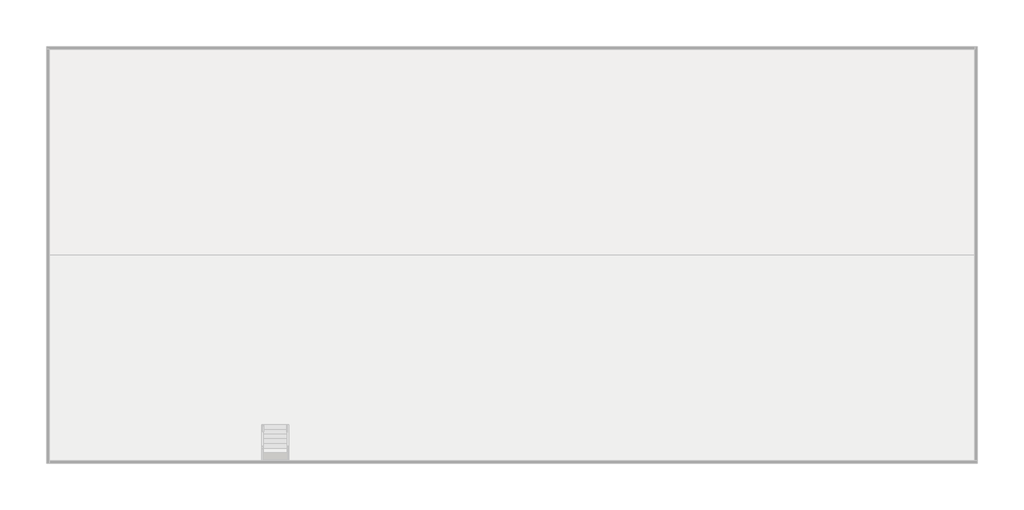
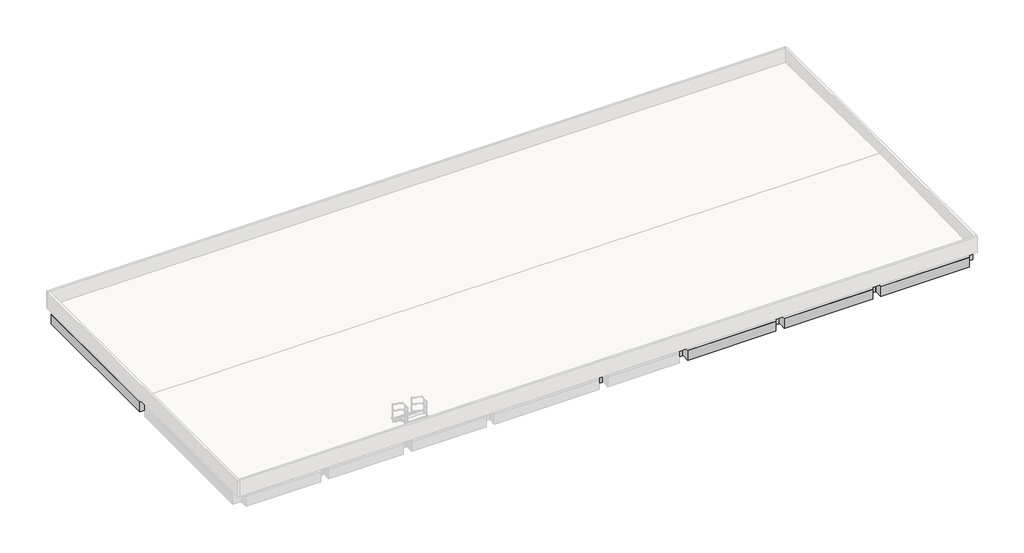
# One storey, part 2 of 3: 33 beams.
"""IFC4 building model written with IfcOpenShell, lengths in millimetres."""

from ifc_helpers import new_model, si_unit, origin, place, context, project, spatial, faceted_brep, element, save

model = new_model("IFC4")

# Units and contexts
model_context = context("Model", 3, world=origin())
ifc_project = project(units=[si_unit("LENGTHUNIT", "METRE", prefix="MILLI")], contexts=[model_context])

# Site, building, storey
site = spatial("IfcSite", under=ifc_project)
building = spatial("IfcBuilding", under=site)
storey = spatial("IfcBuildingStorey", under=building, Name="TOC", Elevation=7499.9618634)

# Beams
placement = place(None, origin())
element("IfcBeam", 1, ObjectType="RC Beam_Rectangular : H_SB_AR_S16_B600xH900_RG9", at=placement, inside=storey, context=model_context, shape_type="Brep", body=[
    faceted_brep([(300.0, 24199.5208589, 6599.9618634), (300.0, 23749.5208589, 6599.9618634), (300.0, 23599.5208589, 6599.9618634), (300.0, 23599.5208589, 7349.9618634), (300.0, 24199.5208589, 7349.9618634), (5700.0, 23599.5208589, 6599.9618634), (5700.0, 23749.5208589, 6599.9618634), (5700.0, 24199.5208589, 6599.9618634), (5700.0, 24199.5208589, 7349.9618634), (5700.0, 23599.5208589, 7349.9618634), (2800.0, 23599.5208589, 7349.9618634), (3200.0, 23599.5208589, 7349.9618634), (2800.0, 23599.5208589, 6599.9618634), (3200.0, 23599.5208589, 6599.9618634)], [[[0, 1, 2, 3, 4]], [[5, 6, 7, 8, 9]], [[4, 3, 10, 11, 9, 8]], [[2, 12, 13, 5, 9, 11, 10, 3]], [[2, 1, 0, 7, 6, 5, 13, 12]], [[7, 0, 4, 8]]]),
])
element("IfcBeam", 2, ObjectType="RC Beam_Rectangular : H_SB_AR_S16_B600xH900_RG9", at=placement, inside=storey, context=model_context, shape_type="Brep", body=[
    faceted_brep([(6300.0, 24199.5208589, 6599.9618634), (6300.0, 23749.5208589, 6599.9618634), (6300.0, 23599.5208589, 6599.9618634), (6300.0, 23599.5208589, 7349.9618634), (6300.0, 24199.5208589, 7349.9618634), (11700.0, 23599.5208589, 6599.9618634), (11700.0, 23749.5208589, 6599.9618634), (11700.0, 24199.5208589, 6599.9618634), (11700.0, 24199.5208589, 7349.9618634), (11700.0, 23599.5208589, 7349.9618634), (8800.0, 23599.5208589, 7349.9618634), (9200.0, 23599.5208589, 7349.9618634), (8800.0, 23599.5208589, 6599.9618634), (9200.0, 23599.5208589, 6599.9618634)], [[[0, 1, 2, 3, 4]], [[5, 6, 7, 8, 9]], [[4, 3, 10, 11, 9, 8]], [[2, 12, 13, 5, 9, 11, 10, 3]], [[2, 1, 0, 7, 6, 5, 13, 12]], [[7, 0, 4, 8]]]),
])
element("IfcBeam", 3, ObjectType="RC Beam_Rectangular : H_SB_AR_S16_B600xH900_RG9", at=placement, inside=storey, context=model_context, shape_type="Brep", body=[
    faceted_brep([(12300.0, 24199.5208589, 6599.9618634), (12300.0, 23749.5208589, 6599.9618634), (12300.0, 23599.5208589, 6599.9618634), (12300.0, 23599.5208589, 7349.9618634), (12300.0, 24199.5208589, 7349.9618634), (17700.0, 23599.5208589, 6599.9618634), (17700.0, 23749.5208589, 6599.9618634), (17700.0, 24199.5208589, 6599.9618634), (17700.0, 24199.5208589, 7349.9618634), (17700.0, 23599.5208589, 7349.9618634), (14800.0, 23599.5208589, 7349.9618634), (15200.0, 23599.5208589, 7349.9618634), (14800.0, 23599.5208589, 6599.9618634), (15200.0, 23599.5208589, 6599.9618634)], [[[0, 1, 2, 3, 4]], [[5, 6, 7, 8, 9]], [[4, 3, 10, 11, 9, 8]], [[2, 12, 13, 5, 9, 11, 10, 3]], [[2, 1, 0, 7, 6, 5, 13, 12]], [[7, 0, 4, 8]]]),
])
element("IfcBeam", 4, ObjectType="RC Beam_Rectangular : H_SB_AR_S16_B600xH900_RG9", at=placement, inside=storey, context=model_context, shape_type="Brep", body=[
    faceted_brep([(18300.0, 24199.5208589, 6599.9618634), (18300.0, 23749.5208589, 6599.9618634), (18300.0, 23599.5208589, 6599.9618634), (18300.0, 23599.5208589, 7349.9618634), (18300.0, 24199.5208589, 7349.9618634), (25900.0, 23599.5208589, 6599.9618634), (25900.0, 23749.5208589, 6599.9618634), (25900.0, 24199.5208589, 6599.9618634), (25900.0, 24199.5208589, 7349.9618634), (25900.0, 23599.5208589, 7349.9618634), (21800.0, 23599.5208589, 7349.9618634), (22400.0, 23599.5208589, 7349.9618634), (21800.0, 23599.5208589, 6599.9618634), (22400.0, 23599.5208589, 6599.9618634)], [[[0, 1, 2, 3, 4]], [[5, 6, 7, 8, 9]], [[4, 3, 10, 11, 9, 8]], [[2, 12, 13, 5, 9, 11, 10, 3]], [[2, 1, 0, 7, 6, 5, 13, 12]], [[7, 0, 4, 8]]]),
])
element("IfcBeam", 5, ObjectType="RC Beam_Rectangular : H_SB_AR_S16_B600xH900_RG9", at=placement, inside=storey, context=model_context, shape_type="Brep", body=[
    faceted_brep([(26500.0, 24199.5208589, 6599.9618634), (26500.0, 23749.5208589, 6599.9618634), (26500.0, 23599.5208589, 6599.9618634), (26500.0, 23599.5208589, 7349.9618634), (26500.0, 24199.5208589, 7349.9618634), (31700.0, 23599.5208589, 6599.9618634), (31700.0, 23749.5208589, 6599.9618634), (31700.0, 24199.5208589, 6599.9618634), (31700.0, 24199.5208589, 7349.9618634), (31700.0, 23599.5208589, 7349.9618634), (28800.0, 23599.5208589, 7349.9618634), (29400.0, 23599.5208589, 7349.9618634), (28800.0, 23599.5208589, 6599.9618634), (29400.0, 23599.5208589, 6599.9618634)], [[[0, 1, 2, 3, 4]], [[5, 6, 7, 8, 9]], [[4, 3, 10, 11, 9, 8]], [[2, 12, 13, 5, 9, 11, 10, 3]], [[2, 1, 0, 7, 6, 5, 13, 12]], [[7, 0, 4, 8]]]),
])
element("IfcBeam", 6, ObjectType="RC Beam_Rectangular : H_SB_AR_S16_B600xH900_RG5", at=placement, inside=storey, context=model_context, shape_type="Brep", body=[
    faceted_brep([(26500.0, 8599.5208589, 6599.9618634), (26500.0, 8399.5208589, 6599.9618634), (26500.0, 7999.5208589, 6599.9618634), (26500.0, 7999.5208589, 7349.9618634), (26500.0, 8599.5208589, 7349.9618634), (31700.0, 7999.5208589, 6599.9618634), (31700.0, 8399.5208589, 6599.9618634), (31700.0, 8599.5208589, 6599.9618634), (31700.0, 8599.5208589, 7349.9618634), (31700.0, 7999.5208589, 7349.9618634), (28500.0, 7999.5208589, 7349.9618634), (28700.0, 7999.5208589, 7349.9618634), (28800.0, 7999.5208589, 7349.9618634), (29400.0, 7999.5208589, 7349.9618634), (29400.0, 8599.5208589, 7349.9618634), (28800.0, 8599.5208589, 7349.9618634), (28500.0, 7999.5208589, 6599.9618634), (28700.0, 7999.5208589, 6599.9618634), (28800.0, 7999.5208589, 6599.9618634), (29400.0, 7999.5208589, 6599.9618634), (28800.0, 8599.5208589, 6599.9618634), (29400.0, 8599.5208589, 6599.9618634)], [[[0, 1, 2, 3, 4]], [[5, 6, 7, 8, 9]], [[4, 3, 10, 11, 12, 13, 9, 8, 14, 15]], [[2, 16, 17, 18, 19, 5, 9, 13, 12, 11, 10, 3]], [[2, 1, 0, 20, 21, 7, 6, 5, 19, 18, 17, 16]], [[7, 21, 20, 0, 4, 15, 14, 8]]]),
])
element("IfcBeam", 7, ObjectType="RC Beam_Rectangular : H_SB_AR_S16_B600xH900_RG5", at=placement, inside=storey, context=model_context, shape_type="Brep", body=[
    faceted_brep([(32300.0, 8599.5208589, 6599.9618634), (32300.0, 8399.5208589, 6599.9618634), (32300.0, 7999.5208589, 6599.9618634), (32300.0, 7999.5208589, 7349.9618634), (32300.0, 8599.5208589, 7349.9618634), (38700.0, 7999.5208589, 6599.9618634), (38700.0, 8599.5208589, 6599.9618634), (38700.0, 8599.5208589, 7349.9618634), (38700.0, 7999.5208589, 7349.9618634), (35200.0, 7999.5208589, 7349.9618634), (35800.0, 7999.5208589, 7349.9618634), (36500.0, 7999.5208589, 7349.9618634), (36700.0, 7999.5208589, 7349.9618634), (36700.0, 8599.5208589, 7349.9618634), (36500.0, 8599.5208589, 7349.9618634), (35800.0, 8599.5208589, 7349.9618634), (35200.0, 8599.5208589, 7349.9618634), (33450.0, 8599.5208589, 7349.9618634), (33250.0, 8599.5208589, 7349.9618634), (35200.0, 7999.5208589, 6599.9618634), (35800.0, 7999.5208589, 6599.9618634), (36500.0, 7999.5208589, 6599.9618634), (36700.0, 7999.5208589, 6599.9618634), (35200.0, 8599.5208589, 6599.9618634), (35800.0, 8599.5208589, 6599.9618634), (36500.0, 8599.5208589, 6599.9618634), (36700.0, 8599.5208589, 6599.9618634)], [[[0, 1, 2, 3, 4]], [[5, 6, 7, 8]], [[4, 3, 9, 10, 11, 12, 8, 7, 13, 14, 15, 16, 17, 18]], [[2, 19, 20, 21, 22, 5, 8, 12, 11, 10, 9, 3]], [[2, 1, 0, 23, 24, 25, 26, 6, 5, 22, 21, 20, 19]], [[6, 26, 25, 24, 23, 0, 4, 18, 17, 16, 15, 14, 13, 7]]]),
])
element("IfcBeam", 8, ObjectType="RC Beam_Rectangular : H_SB_AR_S16_B600xH900_RG5", at=placement, inside=storey, context=model_context, shape_type="Brep", body=[
    faceted_brep([(39300.0, 8599.5208589, 6599.9618634), (39300.0, 8404.5208589, 6599.9618634), (39300.0, 8204.5208589, 6599.9618634), (39300.0, 7999.5208589, 6599.9618634), (39300.0, 7999.5208589, 7349.9618634), (39300.0, 8599.5208589, 7349.9618634), (45700.0, 7999.5208589, 6599.9618634), (45700.0, 8399.5208589, 6599.9618634), (45700.0, 8599.5208589, 6599.9618634), (45700.0, 8599.5208589, 7349.9618634), (45700.0, 7999.5208589, 7349.9618634), (41925.0, 7999.5208589, 7349.9618634), (42125.0, 7999.5208589, 7349.9618634), (42200.0, 7999.5208589, 7349.9618634), (42800.0, 7999.5208589, 7349.9618634), (43200.0, 7999.5208589, 7349.9618634), (43400.0, 7999.5208589, 7349.9618634), (42800.0, 8599.5208589, 7349.9618634), (42200.0, 8599.5208589, 7349.9618634), (41925.0, 7999.5208589, 6599.9618634), (42125.0, 7999.5208589, 6599.9618634), (42200.0, 7999.5208589, 6599.9618634), (42800.0, 7999.5208589, 6599.9618634), (43200.0, 7999.5208589, 6599.9618634), (43400.0, 7999.5208589, 6599.9618634), (42200.0, 8599.5208589, 6599.9618634), (42800.0, 8599.5208589, 6599.9618634), (45640.0, 8599.5208589, 6599.9618634)], [[[0, 1, 2, 3, 4, 5]], [[6, 7, 8, 9, 10]], [[5, 4, 11, 12, 13, 14, 15, 16, 10, 9, 17, 18]], [[3, 19, 20, 21, 22, 23, 24, 6, 10, 16, 15, 14, 13, 12, 11, 4]], [[3, 2, 1, 0, 25, 26, 27, 8, 7, 6, 24, 23, 22, 21, 20, 19]], [[8, 27, 26, 25, 0, 5, 18, 17, 9]]]),
])
element("IfcBeam", 9, ObjectType="RC Beam_Rectangular : H_SB_AR_S16_B600xH900_RG5", at=placement, inside=storey, context=model_context, shape_type="Brep", body=[
    faceted_brep([(46300.0, 8599.5208589, 6599.9618634), (46300.0, 8399.5208589, 6599.9618634), (46300.0, 7999.5208589, 6599.9618634), (46300.0, 7999.5208589, 7349.9618634), (46300.0, 8599.5208589, 7349.9618634), (52700.0, 7999.5208589, 6599.9618634), (52700.0, 8399.5208589, 6599.9618634), (52700.0, 8599.5208589, 6599.9618634), (52700.0, 8599.5208589, 7349.9618634), (52700.0, 7999.5208589, 7349.9618634), (49200.0, 7999.5208589, 7349.9618634), (49800.0, 7999.5208589, 7349.9618634), (52574.0, 7999.5208589, 7349.9618634), (52574.0, 8599.5208589, 7349.9618634), (50725.0, 8599.5208589, 7349.9618634), (50525.0, 8599.5208589, 7349.9618634), (49800.0, 8599.5208589, 7349.9618634), (49200.0, 8599.5208589, 7349.9618634), (49200.0, 7999.5208589, 6599.9618634), (49800.0, 7999.5208589, 6599.9618634), (52574.0, 7999.5208589, 6599.9618634), (49200.0, 8599.5208589, 6599.9618634), (49800.0, 8599.5208589, 6599.9618634)], [[[0, 1, 2, 3, 4]], [[5, 6, 7, 8, 9]], [[4, 3, 10, 11, 12, 9, 8, 13, 14, 15, 16, 17]], [[2, 18, 19, 20, 5, 9, 12, 11, 10, 3]], [[2, 1, 0, 21, 22, 7, 6, 5, 20, 19, 18]], [[7, 22, 21, 0, 4, 17, 16, 15, 14, 13, 8]]]),
])
element("IfcBeam", 10, ObjectType="RC Beam_Rectangular : H_SB_AR_S16_B600xH900_RG9", at=placement, inside=storey, context=model_context, shape_type="Brep", body=[
    faceted_brep([(32300.0, 799.5208589, 6599.9618634), (32300.0, 649.5208589, 6599.9618634), (32300.0, 199.5208589, 6599.9618634), (32300.0, 199.5208589, 7349.9618634), (32300.0, 799.5208589, 7349.9618634), (38700.0, 199.5208589, 6599.9618634), (38700.0, 649.5208589, 6599.9618634), (38700.0, 799.5208589, 6599.9618634), (38700.0, 799.5208589, 7349.9618634), (38700.0, 199.5208589, 7349.9618634), (36700.0, 799.5208589, 7349.9618634), (36500.0, 799.5208589, 7349.9618634), (35800.0, 799.5208589, 7349.9618634), (35200.0, 799.5208589, 7349.9618634), (35200.0, 799.5208589, 6599.9618634), (35800.0, 799.5208589, 6599.9618634)], [[[0, 1, 2, 3, 4]], [[5, 6, 7, 8, 9]], [[4, 3, 9, 8, 10, 11, 12, 13]], [[2, 5, 9, 3]], [[2, 1, 0, 14, 15, 7, 6, 5]], [[7, 15, 14, 0, 4, 13, 12, 11, 10, 8]]]),
])
element("IfcBeam", 11, ObjectType="RC Beam_Rectangular : H_SB_AR_S16_B600xH900_RG9", at=placement, inside=storey, context=model_context, shape_type="Brep", body=[
    faceted_brep([(39300.0, 799.5208589, 6599.9618634), (39300.0, 649.5208589, 6599.9618634), (39300.0, 199.5208589, 6599.9618634), (39300.0, 199.5208589, 7349.9618634), (39300.0, 799.5208589, 7349.9618634), (45700.0, 199.5208589, 6599.9618634), (45700.0, 649.5208589, 6599.9618634), (45700.0, 799.5208589, 6599.9618634), (45700.0, 799.5208589, 7349.9618634), (45700.0, 199.5208589, 7349.9618634), (43400.0, 799.5208589, 7349.9618634), (43200.0, 799.5208589, 7349.9618634), (42800.0, 799.5208589, 7349.9618634), (42200.0, 799.5208589, 7349.9618634), (42200.0, 799.5208589, 6599.9618634), (42800.0, 799.5208589, 6599.9618634)], [[[0, 1, 2, 3, 4]], [[5, 6, 7, 8, 9]], [[4, 3, 9, 8, 10, 11, 12, 13]], [[2, 5, 9, 3]], [[2, 1, 0, 14, 15, 7, 6, 5]], [[7, 15, 14, 0, 4, 13, 12, 11, 10, 8]]]),
])
element("IfcBeam", 12, ObjectType="RC Beam_Rectangular : H_SB_AR_S16_B600xH900_RG9", at=placement, inside=storey, context=model_context, shape_type="Brep", body=[
    faceted_brep([(46300.0, 799.5208589, 6599.9618634), (46300.0, 649.5208589, 6599.9618634), (46300.0, 199.5208589, 6599.9618634), (46300.0, 199.5208589, 7349.9618634), (46300.0, 799.5208589, 7349.9618634), (52700.0, 199.5208589, 6599.9618634), (52700.0, 649.5208589, 6599.9618634), (52700.0, 799.5208589, 6599.9618634), (52700.0, 799.5208589, 7349.9618634), (52700.0, 199.5208589, 7349.9618634), (49800.0, 799.5208589, 7349.9618634), (49200.0, 799.5208589, 7349.9618634), (46800.0, 799.5208589, 7349.9618634), (46600.0, 799.5208589, 7349.9618634), (49200.0, 799.5208589, 6599.9618634), (49800.0, 799.5208589, 6599.9618634)], [[[0, 1, 2, 3, 4]], [[5, 6, 7, 8, 9]], [[4, 3, 9, 8, 10, 11, 12, 13]], [[2, 5, 9, 3]], [[2, 1, 0, 14, 15, 7, 6, 5]], [[7, 15, 14, 0, 4, 13, 12, 11, 10, 8]]]),
])
element("IfcBeam", 13, ObjectType="RC Beam_Rectangular : H_SB_AR_S16_B600xH900_RG6", at=placement, inside=storey, context=model_context, shape_type="Brep", body=[
    faceted_brep([(-300.0, 12499.5208589, 6599.9618634), (150.0, 12499.5208589, 6599.9618634), (300.0, 12499.5208589, 6599.9618634), (300.0, 12499.5208589, 7349.9618634), (-300.0, 12499.5208589, 7349.9618634), (300.0, 23599.5208589, 6599.9618634), (150.0, 23599.5208589, 6599.9618634), (-300.0, 23599.5208589, 6599.9618634), (-300.0, 23599.5208589, 7349.9618634), (300.0, 23599.5208589, 7349.9618634), (300.0, 23473.5208589, 7349.9618634)], [[[0, 1, 2, 3, 4]], [[5, 6, 7, 8, 9]], [[4, 3, 10, 9, 8]], [[2, 5, 9, 10, 3]], [[2, 1, 0, 7, 6, 5]], [[7, 0, 4, 8]]]),
])
element("IfcBeam", 14, ObjectType="RC Beam_Rectangular : H_SB_AR_S16_B400xH900_RG1", at=placement, inside=storey, context=model_context, shape_type="Brep", body=[
    faceted_brep([(6200.0, 23599.5208589, 7349.9618634), (5800.0, 23599.5208589, 7349.9618634), (5800.0, 23473.5208589, 7349.9618634), (5800.0, 12499.5208589, 7349.9618634), (6200.0, 12499.5208589, 7349.9618634), (6200.0, 23473.5208589, 7349.9618634), (6200.0, 23599.5208589, 6599.9618634), (5800.0, 23599.5208589, 6599.9618634), (5800.0, 12499.5208589, 6599.9618634), (6200.0, 12499.5208589, 6599.9618634), (6200.0, 23473.5208589, 6599.9618634), (5800.0, 23473.5208589, 6599.9618634)], [[[0, 1, 2, 3, 4, 5]], [[6, 7, 1, 0]], [[8, 9, 4, 3]], [[9, 10, 6, 0, 5, 4]], [[8, 11, 7, 6, 10, 9]], [[7, 11, 8, 3, 2, 1]]]),
])
element("IfcBeam", 15, ObjectType="RC Beam_Rectangular : H_SB_AR_S16_B400xH900_RG1", at=placement, inside=storey, context=model_context, shape_type="Brep", body=[
    faceted_brep([(12200.0, 23599.5208589, 7349.9618634), (11800.0, 23599.5208589, 7349.9618634), (11800.0, 23473.5208589, 7349.9618634), (11800.0, 12499.5208589, 7349.9618634), (12200.0, 12499.5208589, 7349.9618634), (12200.0, 23473.5208589, 7349.9618634), (12200.0, 23599.5208589, 6599.9618634), (11800.0, 23599.5208589, 6599.9618634), (11800.0, 12499.5208589, 6599.9618634), (12200.0, 12499.5208589, 6599.9618634), (12200.0, 23473.5208589, 6599.9618634), (11800.0, 23473.5208589, 6599.9618634)], [[[0, 1, 2, 3, 4, 5]], [[6, 7, 1, 0]], [[8, 9, 4, 3]], [[9, 10, 6, 0, 5, 4]], [[9, 8, 11, 7, 6, 10]], [[7, 11, 8, 3, 2, 1]]]),
])
element("IfcBeam", 16, ObjectType="RC Beam_Rectangular : H_SB_AR_S16_B600xH900_RG1A", at=placement, inside=storey, context=model_context, shape_type="Brep", body=[
    faceted_brep([(17700.0, 12499.5208589, 6599.9618634), (18100.0, 12499.5208589, 6599.9618634), (18300.0, 12499.5208589, 6599.9618634), (18300.0, 12499.5208589, 7349.9618634), (17700.0, 12499.5208589, 7349.9618634), (18300.0, 23473.5208589, 7349.9618634), (18300.0, 23599.5208589, 7349.9618634), (17700.0, 23599.5208589, 7349.9618634), (17700.0, 23473.5208589, 7349.9618634), (18300.0, 23599.5208589, 6599.9618634), (18100.0, 23599.5208589, 6599.9618634), (17700.0, 23599.5208589, 6599.9618634), (17700.0, 23473.5208589, 6599.9618634)], [[[0, 1, 2, 3, 4]], [[4, 3, 5, 6, 7, 8]], [[9, 10, 11, 7, 6]], [[2, 9, 6, 5, 3]], [[0, 12, 11, 10, 9, 2, 1]], [[11, 12, 0, 4, 8, 7]]]),
])
element("IfcBeam", 17, ObjectType="RC Beam_Rectangular : H_SB_AR_S16_B500xH900_RG3", at=placement, inside=storey, context=model_context, shape_type="Brep", body=[
    faceted_brep([(26450.0, 7999.5208589, 6599.9618634), (26300.0, 7999.5208589, 6599.9618634), (26100.0, 7999.5208589, 6599.9618634), (25950.0, 7999.5208589, 6599.9618634), (25950.0, 7999.5208589, 7349.9618634), (26450.0, 7999.5208589, 7349.9618634), (25950.0, 925.5208589, 7349.9618634), (25950.0, 799.5208589, 7349.9618634), (26450.0, 799.5208589, 7349.9618634), (26450.0, 925.5208589, 7349.9618634), (26450.0, 2637.0208589, 7349.9618634), (26450.0, 2837.0208589, 7349.9618634), (25950.0, 799.5208589, 6599.9618634), (26100.0, 799.5208589, 6599.9618634), (26300.0, 799.5208589, 6599.9618634), (26450.0, 799.5208589, 6599.9618634), (26450.0, 925.5208589, 6599.9618634), (26450.0, 2637.0208589, 6599.9618634), (26450.0, 2837.0208589, 6599.9618634), (25950.0, 925.5208589, 6599.9618634)], [[[0, 1, 2, 3, 4, 5]], [[5, 4, 6, 7, 8, 9, 10, 11]], [[12, 13, 14, 15, 8, 7]], [[15, 16, 17, 18, 0, 5, 11, 10, 9, 8]], [[12, 19, 3, 2, 1, 0, 18, 17, 16, 15, 14, 13]], [[3, 19, 12, 7, 6, 4]]]),
])
element("IfcBeam", 18, ObjectType="RC Beam_Rectangular : H_SB_AR_S16_B500xH900_RG2", at=placement, inside=storey, context=model_context, shape_type="Brep", body=[
    faceted_brep([(26450.0, 23599.5208589, 7349.9618634), (25950.0, 23599.5208589, 7349.9618634), (25950.0, 23473.5208589, 7349.9618634), (25950.0, 8599.5208589, 7349.9618634), (26450.0, 8599.5208589, 7349.9618634), (26450.0, 23473.5208589, 7349.9618634), (26450.0, 23599.5208589, 6599.9618634), (25950.0, 23599.5208589, 6599.9618634), (25950.0, 8599.5208589, 6599.9618634), (26450.0, 8599.5208589, 6599.9618634), (26450.0, 23473.5208589, 6599.9618634), (25950.0, 23473.5208589, 6599.9618634)], [[[0, 1, 2, 3, 4, 5]], [[6, 7, 1, 0]], [[8, 9, 4, 3]], [[9, 10, 6, 0, 5, 4]], [[6, 10, 9, 8, 11, 7]], [[7, 11, 8, 3, 2, 1]]]),
])
element("IfcBeam", 19, ObjectType="RC Beam_Rectangular : H_SB_AR_S16_B500xH900_RG3", at=placement, inside=storey, context=model_context, shape_type="Brep", body=[
    faceted_brep([(31750.0, 799.5208589, 7349.9618634), (32250.0, 799.5208589, 7349.9618634), (32250.0, 925.5208589, 7349.9618634), (32250.0, 7999.5208589, 7349.9618634), (31750.0, 7999.5208589, 7349.9618634), (31750.0, 799.5208589, 6599.9618634), (31900.0, 799.5208589, 6599.9618634), (32250.0, 799.5208589, 6599.9618634), (32250.0, 7999.5208589, 6599.9618634), (31900.0, 7999.5208589, 6599.9618634), (31750.0, 7999.5208589, 6599.9618634), (32250.0, 925.5208589, 6599.9618634)], [[[0, 1, 2, 3, 4]], [[5, 6, 7, 1, 0]], [[8, 9, 10, 4, 3]], [[7, 11, 8, 3, 2, 1]], [[5, 10, 9, 8, 11, 7, 6]], [[10, 5, 0, 4]]]),
])
element("IfcBeam", 20, ObjectType="RC Beam_Rectangular : H_SB_AR_S16_B500xH900_RG2", at=placement, inside=storey, context=model_context, shape_type="Brep", body=[
    faceted_brep([(32250.0, 23599.5208589, 7349.9618634), (31750.0, 23599.5208589, 7349.9618634), (31750.0, 23473.5208589, 7349.9618634), (31750.0, 8599.5208589, 7349.9618634), (32250.0, 8599.5208589, 7349.9618634), (32250.0, 23473.5208589, 7349.9618634), (32250.0, 23599.5208589, 6599.9618634), (31750.0, 23599.5208589, 6599.9618634), (31750.0, 8599.5208589, 6599.9618634), (32250.0, 8599.5208589, 6599.9618634), (32250.0, 23473.5208589, 6599.9618634), (31750.0, 23473.5208589, 6599.9618634)], [[[0, 1, 2, 3, 4, 5]], [[6, 7, 1, 0]], [[8, 9, 4, 3]], [[9, 10, 6, 0, 5, 4]], [[8, 11, 7, 6, 10, 9]], [[7, 11, 8, 3, 2, 1]]]),
])
element("IfcBeam", 21, ObjectType="RC Beam_Rectangular : H_SB_AR_S16_B500xH900_RG3", at=placement, inside=storey, context=model_context, shape_type="Brep", body=[
    faceted_brep([(38750.0, 799.5208589, 7349.9618634), (39250.0, 799.5208589, 7349.9618634), (39250.0, 925.5208589, 7349.9618634), (39250.0, 4649.5208589, 7349.9618634), (39250.0, 4849.5208589, 7349.9618634), (39250.0, 7999.5208589, 7349.9618634), (38750.0, 7999.5208589, 7349.9618634), (38750.0, 3543.8249516, 7349.9618634), (38750.0, 3343.8249516, 7349.9618634), (38750.0, 925.5208589, 7349.9618634), (38750.0, 799.5208589, 6599.9618634), (38900.0, 799.5208589, 6599.9618634), (39100.0, 799.5208589, 6599.9618634), (39250.0, 799.5208589, 6599.9618634), (39250.0, 7999.5208589, 6599.9618634), (39100.0, 7999.5208589, 6599.9618634), (38900.0, 7999.5208589, 6599.9618634), (38750.0, 7999.5208589, 6599.9618634), (39250.0, 925.5208589, 6599.9618634), (39250.0, 4649.5208589, 6599.9618634), (39250.0, 4849.5208589, 6599.9618634), (38750.0, 925.5208589, 6599.9618634), (38750.0, 3343.8249516, 6599.9618634), (38750.0, 3543.8249516, 6599.9618634)], [[[0, 1, 2, 3, 4, 5, 6, 7, 8, 9]], [[10, 11, 12, 13, 1, 0]], [[14, 15, 16, 17, 6, 5]], [[13, 18, 19, 20, 14, 5, 4, 3, 2, 1]], [[10, 21, 22, 23, 17, 16, 15, 14, 20, 19, 18, 13, 12, 11]], [[17, 23, 22, 21, 10, 0, 9, 8, 7, 6]]]),
])
element("IfcBeam", 22, ObjectType="RC Beam_Rectangular : H_SB_AR_S16_B500xH900_RG3", at=placement, inside=storey, context=model_context, shape_type="Brep", body=[
    faceted_brep([(45750.0, 799.5208589, 7349.9618634), (46250.0, 799.5208589, 7349.9618634), (46250.0, 925.5208589, 7349.9618634), (46250.0, 4649.5208589, 7349.9618634), (46250.0, 4849.5208589, 7349.9618634), (46250.0, 6599.5208589, 7349.9618634), (46250.0, 6799.5208589, 7349.9618634), (46250.0, 7999.5208589, 7349.9618634), (45750.0, 7999.5208589, 7349.9618634), (45750.0, 6799.5208589, 7349.9618634), (45750.0, 6599.5208589, 7349.9618634), (45750.0, 4849.5208589, 7349.9618634), (45750.0, 4649.5208589, 7349.9618634), (45750.0, 925.5208589, 7349.9618634), (45750.0, 799.5208589, 6599.9618634), (46250.0, 799.5208589, 6599.9618634), (46250.0, 7999.5208589, 6599.9618634), (45750.0, 7999.5208589, 6599.9618634), (46250.0, 925.5208589, 6599.9618634), (46250.0, 4649.5208589, 6599.9618634), (46250.0, 4849.5208589, 6599.9618634), (46250.0, 6599.5208589, 6599.9618634), (46250.0, 6799.5208589, 6599.9618634), (45750.0, 925.5208589, 6599.9618634), (45750.0, 4649.5208589, 6599.9618634), (45750.0, 4849.5208589, 6599.9618634), (45750.0, 6599.5208589, 6599.9618634), (45750.0, 6799.5208589, 6599.9618634)], [[[0, 1, 2, 3, 4, 5, 6, 7, 8, 9, 10, 11, 12, 13]], [[14, 15, 1, 0]], [[16, 17, 8, 7]], [[15, 18, 19, 20, 21, 22, 16, 7, 6, 5, 4, 3, 2, 1]], [[14, 23, 24, 25, 26, 27, 17, 16, 22, 21, 20, 19, 18, 15]], [[17, 27, 26, 25, 24, 23, 14, 0, 13, 12, 11, 10, 9, 8]]]),
])
element("IfcBeam", 23, ObjectType="RC Beam_Rectangular : H_SB_AR_S16_B600xH900_RG8", at=placement, inside=storey, context=model_context, shape_type="Brep", body=[
    faceted_brep([(53300.0, 7999.5208589, 6599.9618634), (52850.0, 7999.5208589, 6599.9618634), (52700.0, 7999.5208589, 6599.9618634), (52700.0, 7999.5208589, 7349.9618634), (53300.0, 7999.5208589, 7349.9618634), (52700.0, 799.5208589, 6599.9618634), (52850.0, 799.5208589, 6599.9618634), (53300.0, 799.5208589, 6599.9618634), (53300.0, 799.5208589, 7349.9618634), (52700.0, 799.5208589, 7349.9618634), (52700.0, 925.5208589, 7349.9618634)], [[[0, 1, 2, 3, 4]], [[5, 6, 7, 8, 9]], [[4, 3, 10, 9, 8]], [[7, 0, 4, 8]], [[2, 1, 0, 7, 6, 5]], [[2, 5, 9, 10, 3]]]),
])
element("IfcBeam", 24, ObjectType="RC Beam_Rectangular : H_SB_AR_S16_B600xH900_RG5A", at=placement, inside=storey, context=model_context, shape_type="Brep", body=[
    faceted_brep([(18300.0, 7999.5208589, 6599.9618634), (21800.0, 7999.5208589, 6599.9618634), (22400.0, 7999.5208589, 6599.9618634), (25900.0, 7999.5208589, 6599.9618634), (25900.0, 7999.5208589, 7349.9618634), (22400.0, 7999.5208589, 7349.9618634), (21800.0, 7999.5208589, 7349.9618634), (18300.0, 7999.5208589, 7349.9618634), (25900.0, 8599.5208589, 6599.9618634), (25900.0, 8399.5208589, 6599.9618634), (18300.0, 8399.5208589, 6599.9618634), (18300.0, 8599.5208589, 6599.9618634), (21800.0, 8599.5208589, 6599.9618634), (22400.0, 8599.5208589, 6599.9618634), (18300.0, 8599.5208589, 7349.9618634), (21800.0, 8599.5208589, 7349.9618634), (22400.0, 8599.5208589, 7349.9618634), (25900.0, 8599.5208589, 7349.9618634)], [[[0, 1, 2, 3, 4, 5, 6, 7]], [[8, 9, 3, 2, 1, 0, 10, 11, 12, 13]], [[8, 13, 12, 11, 14, 15, 16, 17]], [[3, 9, 8, 17, 4]], [[7, 6, 5, 4, 17, 16, 15, 14]], [[11, 10, 0, 7, 14]]]),
])
element("IfcBeam", 25, ObjectType="RC Beam_Rectangular : H_SB_AR_S16_B400xH900_RB1", at=placement, inside=storey, context=model_context, shape_type="Brep", body=[
    faceted_brep([(2800.0, 23599.5208589, 6599.9618634), (2800.0, 23473.5208589, 6599.9618634), (2800.0, 12499.5208589, 6599.9618634), (2800.0, 12499.5208589, 7349.9618634), (2800.0, 23473.5208589, 7349.9618634), (2800.0, 23599.5208589, 7349.9618634), (3200.0, 12499.5208589, 6599.9618634), (3200.0, 23599.5208589, 6599.9618634), (3200.0, 23473.5208589, 6599.9618634), (3200.0, 23599.5208589, 7349.9618634), (3200.0, 23473.5208589, 7349.9618634), (3200.0, 12499.5208589, 7349.9618634)], [[[0, 1, 2, 3, 4, 5]], [[6, 2, 1, 0, 7, 8]], [[6, 8, 7, 9, 10, 11]], [[2, 6, 11, 3]], [[7, 0, 5, 9]], [[5, 4, 3, 11, 10, 9]]]),
])
element("IfcBeam", 26, ObjectType="RC Beam_Rectangular : H_SB_AR_S16_B400xH900_RB1", at=placement, inside=storey, context=model_context, shape_type="Brep", body=[
    faceted_brep([(8800.0, 23599.5208589, 6599.9618634), (8800.0, 23473.5208589, 6599.9618634), (8800.0, 12499.5208589, 6599.9618634), (8800.0, 12499.5208589, 7349.9618634), (8800.0, 23473.5208589, 7349.9618634), (8800.0, 23599.5208589, 7349.9618634), (9200.0, 12499.5208589, 6599.9618634), (9200.0, 23599.5208589, 6599.9618634), (9200.0, 23473.5208589, 6599.9618634), (9200.0, 23599.5208589, 7349.9618634), (9200.0, 23473.5208589, 7349.9618634), (9200.0, 12499.5208589, 7349.9618634)], [[[0, 1, 2, 3, 4, 5]], [[6, 2, 1, 0, 7, 8]], [[6, 8, 7, 9, 10, 11]], [[2, 6, 11, 3]], [[7, 0, 5, 9]], [[5, 4, 3, 11, 10, 9]]]),
])
element("IfcBeam", 27, ObjectType="RC Beam_Rectangular : H_SB_AR_S16_B400xH900_RB1", at=placement, inside=storey, context=model_context, shape_type="Brep", body=[
    faceted_brep([(14800.0, 23599.5208589, 6599.9618634), (14800.0, 23473.5208589, 6599.9618634), (14800.0, 12499.5208589, 6599.9618634), (14800.0, 12499.5208589, 7349.9618634), (14800.0, 23473.5208589, 7349.9618634), (14800.0, 23599.5208589, 7349.9618634), (15200.0, 12499.5208589, 6599.9618634), (15200.0, 23599.5208589, 6599.9618634), (15200.0, 23473.5208589, 6599.9618634), (15200.0, 23599.5208589, 7349.9618634), (15200.0, 23473.5208589, 7349.9618634), (15200.0, 12499.5208589, 7349.9618634)], [[[0, 1, 2, 3, 4, 5]], [[6, 2, 1, 0, 7, 8]], [[6, 8, 7, 9, 10, 11]], [[2, 6, 11, 3]], [[7, 0, 5, 9]], [[5, 4, 3, 11, 10, 9]]]),
])
element("IfcBeam", 28, ObjectType="RC Beam_Rectangular : H_SB_AR_S16_B600xH900_RB2", at=placement, inside=storey, context=model_context, shape_type="Brep", body=[
    faceted_brep([(21800.0, 23599.5208589, 6599.9618634), (21800.0, 23473.5208589, 6599.9618634), (21800.0, 8599.5208589, 6599.9618634), (21800.0, 8599.5208589, 7349.9618634), (21800.0, 23473.5208589, 7349.9618634), (21800.0, 23599.5208589, 7349.9618634), (22400.0, 8599.5208589, 6599.9618634), (22400.0, 23599.5208589, 6599.9618634), (22400.0, 23473.5208589, 6599.9618634), (22400.0, 23599.5208589, 7349.9618634), (22400.0, 23473.5208589, 7349.9618634), (22400.0, 8599.5208589, 7349.9618634)], [[[0, 1, 2, 3, 4, 5]], [[6, 2, 1, 0, 7, 8]], [[6, 8, 7, 9, 10, 11]], [[2, 6, 11, 3]], [[7, 0, 5, 9]], [[5, 4, 3, 11, 10, 9]]]),
])
element("IfcBeam", 29, ObjectType="RC Beam_Rectangular : H_SB_AR_S16_B600xH900_RB2", at=placement, inside=storey, context=model_context, shape_type="Brep", body=[
    faceted_brep([(28800.0, 23599.5208589, 6599.9618634), (28800.0, 23473.5208589, 6599.9618634), (28800.0, 8599.5208589, 6599.9618634), (28800.0, 8599.5208589, 7349.9618634), (28800.0, 23473.5208589, 7349.9618634), (28800.0, 23599.5208589, 7349.9618634), (29400.0, 8599.5208589, 6599.9618634), (29400.0, 23599.5208589, 6599.9618634), (29400.0, 23473.5208589, 6599.9618634), (29400.0, 23599.5208589, 7349.9618634), (29400.0, 23473.5208589, 7349.9618634), (29400.0, 8599.5208589, 7349.9618634)], [[[0, 1, 2, 3, 4, 5]], [[6, 2, 1, 0, 7, 8]], [[6, 8, 7, 9, 10, 11]], [[2, 6, 11, 3]], [[7, 0, 5, 9]], [[5, 4, 3, 11, 10, 9]]]),
])
element("IfcBeam", 30, ObjectType="RC Beam_Rectangular : H_SB_AR_S16_B600xH900_RB3", at=placement, inside=storey, context=model_context, shape_type="Brep", body=[
    faceted_brep([(28800.0, 7999.5208589, 6599.9618634), (28800.0, 4999.0208589, 6599.9618634), (28800.0, 4799.0208589, 6599.9618634), (28800.0, 925.5208589, 6599.9618634), (28800.0, 799.5208589, 6599.9618634), (28800.0, 799.5208589, 7349.9618634), (28800.0, 925.5208589, 7349.9618634), (28800.0, 4799.0208589, 7349.9618634), (28800.0, 4999.0208589, 7349.9618634), (28800.0, 7999.5208589, 7349.9618634), (29400.0, 7999.5208589, 6599.9618634), (29400.0, 4999.0208589, 6599.9618634), (29400.0, 4799.0208589, 6599.9618634), (29400.0, 925.5208589, 6599.9618634), (29400.0, 799.5208589, 6599.9618634), (29400.0, 7999.5208589, 7349.9618634), (29400.0, 4999.0208589, 7349.9618634), (29400.0, 4799.0208589, 7349.9618634), (29400.0, 925.5208589, 7349.9618634), (29400.0, 799.5208589, 7349.9618634)], [[[0, 1, 2, 3, 4, 5, 6, 7, 8, 9]], [[0, 10, 11, 12, 13, 14, 4, 3, 2, 1]], [[14, 13, 12, 11, 10, 15, 16, 17, 18, 19]], [[10, 0, 9, 15]], [[4, 14, 19, 5]], [[9, 8, 7, 6, 5, 19, 18, 17, 16, 15]]]),
])
element("IfcBeam", 31, ObjectType="RC Beam_Rectangular : H_SB_AR_S16_B600xH900_RB3", at=placement, inside=storey, context=model_context, shape_type="Brep", body=[
    faceted_brep([(35200.0, 7999.5208589, 6599.9618634), (35200.0, 925.5208589, 6599.9618634), (35200.0, 799.5208589, 6599.9618634), (35200.0, 799.5208589, 7349.9618634), (35200.0, 925.5208589, 7349.9618634), (35200.0, 7999.5208589, 7349.9618634), (35800.0, 7999.5208589, 6599.9618634), (35800.0, 925.5208589, 6599.9618634), (35800.0, 799.5208589, 6599.9618634), (35800.0, 7999.5208589, 7349.9618634), (35800.0, 925.5208589, 7349.9618634), (35800.0, 799.5208589, 7349.9618634)], [[[0, 1, 2, 3, 4, 5]], [[0, 6, 7, 8, 2, 1]], [[8, 7, 6, 9, 10, 11]], [[6, 0, 5, 9]], [[2, 8, 11, 3]], [[5, 4, 3, 11, 10, 9]]]),
])
element("IfcBeam", 32, ObjectType="RC Beam_Rectangular : H_SB_AR_S16_B600xH900_RB3", at=placement, inside=storey, context=model_context, shape_type="Brep", body=[
    faceted_brep([(42200.0, 7999.5208589, 6599.9618634), (42200.0, 6274.5208589, 6599.9618634), (42200.0, 6074.5208589, 6599.9618634), (42200.0, 4849.5208589, 6599.9618634), (42200.0, 4649.5208589, 6599.9618634), (42200.0, 925.5208589, 6599.9618634), (42200.0, 799.5208589, 6599.9618634), (42200.0, 799.5208589, 7349.9618634), (42200.0, 925.5208589, 7349.9618634), (42200.0, 4649.5208589, 7349.9618634), (42200.0, 4849.5208589, 7349.9618634), (42200.0, 6074.5208589, 7349.9618634), (42200.0, 6274.5208589, 7349.9618634), (42200.0, 7999.5208589, 7349.9618634), (42800.0, 7999.5208589, 6599.9618634), (42800.0, 6274.5208589, 6599.9618634), (42800.0, 6074.5208589, 6599.9618634), (42800.0, 4849.5208589, 6599.9618634), (42800.0, 4649.5208589, 6599.9618634), (42800.0, 925.5208589, 6599.9618634), (42800.0, 799.5208589, 6599.9618634), (42800.0, 7999.5208589, 7349.9618634), (42800.0, 6274.5208589, 7349.9618634), (42800.0, 6074.5208589, 7349.9618634), (42800.0, 4849.5208589, 7349.9618634), (42800.0, 4649.5208589, 7349.9618634), (42800.0, 925.5208589, 7349.9618634), (42800.0, 799.5208589, 7349.9618634)], [[[0, 1, 2, 3, 4, 5, 6, 7, 8, 9, 10, 11, 12, 13]], [[0, 14, 15, 16, 17, 18, 19, 20, 6, 5, 4, 3, 2, 1]], [[20, 19, 18, 17, 16, 15, 14, 21, 22, 23, 24, 25, 26, 27]], [[14, 0, 13, 21]], [[6, 20, 27, 7]], [[13, 12, 11, 10, 9, 8, 7, 27, 26, 25, 24, 23, 22, 21]]]),
])
element("IfcBeam", 33, ObjectType="RC Beam_Rectangular : H_SB_AR_S16_B600xH900_RB3", at=placement, inside=storey, context=model_context, shape_type="Brep", body=[
    faceted_brep([(49200.0, 7999.5208589, 6599.9618634), (49200.0, 925.5208589, 6599.9618634), (49200.0, 799.5208589, 6599.9618634), (49200.0, 799.5208589, 7349.9618634), (49200.0, 925.5208589, 7349.9618634), (49200.0, 7999.5208589, 7349.9618634), (49800.0, 7999.5208589, 6599.9618634), (49800.0, 925.5208589, 6599.9618634), (49800.0, 799.5208589, 6599.9618634), (49800.0, 7999.5208589, 7349.9618634), (49800.0, 925.5208589, 7349.9618634), (49800.0, 799.5208589, 7349.9618634)], [[[0, 1, 2, 3, 4, 5]], [[0, 6, 7, 8, 2, 1]], [[8, 7, 6, 9, 10, 11]], [[6, 0, 5, 9]], [[2, 8, 11, 3]], [[5, 4, 3, 11, 10, 9]]]),
])

save(model, "model.ifc")

# Revit data of these elements
# Type "RC Beam_Rectangular : H_SB_AR_S16_B600xH900_RG9"
#   H_Q'ty Cal Type Tag = "SB-Q1"
#   H_WM Code_1 = "A03AF032-00010 |  | M3 | Concrete Work | Superstructure Work | Structural Concrete | Cement Type-1 | 20MPa < F'c (Cylinder Strength) ≤ 25MPa |  |  |  | A03AF032-00010 Concrete Work Superstructure Work Structural Concrete  Cement Type-1 20MPa < F'c (Cylinder Strength) ≤ 25MPa      |  F'c (Cylinder Strength) = 24MPa"
#   H_WM Code_2 = "A03AD037-00002 |  | TON | Concrete Work | Substructure Work | Rebar Work | Deformed Bar (Non-Coat.) | 400MPa<Fy≤470MPa |  |  |  | A03AD037-00002 Concrete Work Substructure Work Rebar Work Deformed Bar (Non-Coat.)  400MPa<Fy≤470MPa      | ASTM A615 GRADE 60 (Fy=420MPa)"
#   H_WM Code_3 = "A03AF036-00001 |  | M2 | Concrete Work | Superstructure Work | Form Work (1 time in use) | Flat Form | Dressed Lumber, Plywood or Steel Form(Wood Planks are not Allowed) incl. Chamfer |  |  | A03AF036-00001 Concrete Work Superstructure Work Form Work (1 time in use) Flat Form     Dressed Lumber, Plywood or Steel Form(Wood Planks are not Allowed) incl. Chamfer   |"
#   H_WM Code_4 = "A04AM078-00002 |  | M2 | Finishing Work | Painting Work | Internal Wall Painting | Water Emulsion Paint |  |  |  | A04AM078-00002 Finishing Work Painting Work Internal Wall Painting Water Emulsion Paint        |"
#   중앙부 하부근 = ""
#   중앙부 상부근 = ""
#   중앙부 보조근 = ""
#   중앙부 늑근 = ""
#   외단부 하부근 = ""
#   외단부 상부근 = ""
#   외단부 보조근 = ""
#   외단부 늑근 = ""
#   부호 = "TG3"
#   내단부 하부근 = ""
#   내단부 상부근 = ""
#   내단부 보조근 = ""
#   내단부 늑근 = ""
#   ALL 하부근 = "3-D20"
#   ALL 상부근 = "3-D20"
#   ALL 보조근 = ""
#   ALL 늑근 = "2-D10 @120"
#   Width = 600 mm
#   Height = 900 mm
#   Length [instance default] = 1524 mm
#   b = 600 mm
#   h = 900 mm
#   hec_material3 [instance default] = none
#   hec_material2 [instance default] = none
#   hec_material1 [instance default] = none
#   Structural Material [instance default] = none
#   Assembly Code = ""
# Type "RC Beam_Rectangular : H_SB_AR_S16_B600xH900_RG5"
#   H_Q'ty Cal Type Tag = "SB-Q1"
#   H_WM Code_1 = "A03AF032-00010 |  | M3 | Concrete Work | Superstructure Work | Structural Concrete | Cement Type-1 | 20MPa < F'c (Cylinder Strength) ≤ 25MPa |  |  |  | A03AF032-00010 Concrete Work Superstructure Work Structural Concrete  Cement Type-1 20MPa < F'c (Cylinder Strength) ≤ 25MPa      |  F'c (Cylinder Strength) = 24MPa"
#   H_WM Code_2 = "A03AD037-00002 |  | TON | Concrete Work | Substructure Work | Rebar Work | Deformed Bar (Non-Coat.) | 400MPa<Fy≤470MPa |  |  |  | A03AD037-00002 Concrete Work Substructure Work Rebar Work Deformed Bar (Non-Coat.)  400MPa<Fy≤470MPa      | ASTM A615 GRADE 60 (Fy=420MPa)"
#   H_WM Code_3 = "A03AF036-00001 |  | M2 | Concrete Work | Superstructure Work | Form Work (1 time in use) | Flat Form | Dressed Lumber, Plywood or Steel Form(Wood Planks are not Allowed) incl. Chamfer |  |  | A03AF036-00001 Concrete Work Superstructure Work Form Work (1 time in use) Flat Form     Dressed Lumber, Plywood or Steel Form(Wood Planks are not Allowed) incl. Chamfer   |"
#   H_WM Code_4 = "A04AM078-00002 |  | M2 | Finishing Work | Painting Work | Internal Wall Painting | Water Emulsion Paint |  |  |  | A04AM078-00002 Finishing Work Painting Work Internal Wall Painting Water Emulsion Paint        |"
#   중앙부 하부근 = ""
#   중앙부 상부근 = ""
#   중앙부 보조근 = ""
#   중앙부 늑근 = ""
#   외단부 하부근 = ""
#   외단부 상부근 = ""
#   외단부 보조근 = ""
#   외단부 늑근 = ""
#   부호 = "TG3"
#   내단부 하부근 = ""
#   내단부 상부근 = ""
#   내단부 보조근 = ""
#   내단부 늑근 = ""
#   ALL 하부근 = "3-D20"
#   ALL 상부근 = "3-D20"
#   ALL 보조근 = ""
#   ALL 늑근 = "2-D10 @120"
#   Width = 600 mm
#   Height = 900 mm
#   Length [instance default] = 1524 mm
#   b = 600 mm
#   h = 900 mm
#   hec_material3 [instance default] = none
#   hec_material2 [instance default] = none
#   hec_material1 [instance default] = none
#   Structural Material [instance default] = none
#   Assembly Code = ""
# Type "RC Beam_Rectangular : H_SB_AR_S16_B600xH900_RG6"
#   H_Q'ty Cal Type Tag = "SB-Q1"
#   H_WM Code_1 = "A03AF032-00010 |  | M3 | Concrete Work | Superstructure Work | Structural Concrete | Cement Type-1 | 20MPa < F'c (Cylinder Strength) ≤ 25MPa |  |  |  | A03AF032-00010 Concrete Work Superstructure Work Structural Concrete  Cement Type-1 20MPa < F'c (Cylinder Strength) ≤ 25MPa      |  F'c (Cylinder Strength) = 24MPa"
#   H_WM Code_2 = "A03AD037-00002 |  | TON | Concrete Work | Substructure Work | Rebar Work | Deformed Bar (Non-Coat.) | 400MPa<Fy≤470MPa |  |  |  | A03AD037-00002 Concrete Work Substructure Work Rebar Work Deformed Bar (Non-Coat.)  400MPa<Fy≤470MPa      | ASTM A615 GRADE 60 (Fy=420MPa)"
#   H_WM Code_3 = "A03AF036-00001 |  | M2 | Concrete Work | Superstructure Work | Form Work (1 time in use) | Flat Form | Dressed Lumber, Plywood or Steel Form(Wood Planks are not Allowed) incl. Chamfer |  |  | A03AF036-00001 Concrete Work Superstructure Work Form Work (1 time in use) Flat Form     Dressed Lumber, Plywood or Steel Form(Wood Planks are not Allowed) incl. Chamfer   |"
#   H_WM Code_4 = "A04AM078-00002 |  | M2 | Finishing Work | Painting Work | Internal Wall Painting | Water Emulsion Paint |  |  |  | A04AM078-00002 Finishing Work Painting Work Internal Wall Painting Water Emulsion Paint        |"
#   중앙부 하부근 = ""
#   중앙부 상부근 = ""
#   중앙부 보조근 = ""
#   중앙부 늑근 = ""
#   외단부 하부근 = ""
#   외단부 상부근 = ""
#   외단부 보조근 = ""
#   외단부 늑근 = ""
#   부호 = "TG3"
#   내단부 하부근 = ""
#   내단부 상부근 = ""
#   내단부 보조근 = ""
#   내단부 늑근 = ""
#   ALL 하부근 = "3-D20"
#   ALL 상부근 = "3-D20"
#   ALL 보조근 = ""
#   ALL 늑근 = "2-D10 @120"
#   Width = 600 mm
#   Height = 900 mm
#   Length [instance default] = 1524 mm
#   b = 600 mm
#   h = 900 mm
#   hec_material3 [instance default] = none
#   hec_material2 [instance default] = none
#   hec_material1 [instance default] = none
#   Structural Material [instance default] = none
#   Assembly Code = ""
# Type "RC Beam_Rectangular : H_SB_AR_S16_B400xH900_RG1"
#   H_Q'ty Cal Type Tag = "SB-Q1"
#   H_WM Code_1 = "A03AF032-00010 |  | M3 | Concrete Work | Superstructure Work | Structural Concrete | Cement Type-1 | 20MPa < F'c (Cylinder Strength) ≤ 25MPa |  |  |  | A03AF032-00010 Concrete Work Superstructure Work Structural Concrete  Cement Type-1 20MPa < F'c (Cylinder Strength) ≤ 25MPa      |  F'c (Cylinder Strength) = 24MPa"
#   H_WM Code_2 = "A03AD037-00002 |  | TON | Concrete Work | Substructure Work | Rebar Work | Deformed Bar (Non-Coat.) | 400MPa<Fy≤470MPa |  |  |  | A03AD037-00002 Concrete Work Substructure Work Rebar Work Deformed Bar (Non-Coat.)  400MPa<Fy≤470MPa      | ASTM A615 GRADE 60 (Fy=420MPa)"
#   H_WM Code_3 = "A03AF036-00001 |  | M2 | Concrete Work | Superstructure Work | Form Work (1 time in use) | Flat Form | Dressed Lumber, Plywood or Steel Form(Wood Planks are not Allowed) incl. Chamfer |  |  | A03AF036-00001 Concrete Work Superstructure Work Form Work (1 time in use) Flat Form     Dressed Lumber, Plywood or Steel Form(Wood Planks are not Allowed) incl. Chamfer   |"
#   H_WM Code_4 = "A04AM078-00002 |  | M2 | Finishing Work | Painting Work | Internal Wall Painting | Water Emulsion Paint |  |  |  | A04AM078-00002 Finishing Work Painting Work Internal Wall Painting Water Emulsion Paint        |"
#   중앙부 하부근 = ""
#   중앙부 상부근 = ""
#   중앙부 보조근 = ""
#   중앙부 늑근 = ""
#   외단부 하부근 = ""
#   외단부 상부근 = ""
#   외단부 보조근 = ""
#   외단부 늑근 = ""
#   부호 = "TG3"
#   내단부 하부근 = ""
#   내단부 상부근 = ""
#   내단부 보조근 = ""
#   내단부 늑근 = ""
#   ALL 하부근 = "3-D20"
#   ALL 상부근 = "3-D20"
#   ALL 보조근 = ""
#   ALL 늑근 = "2-D10 @120"
#   Width = 400 mm
#   Height = 900 mm
#   Length [instance default] = 1524 mm
#   b = 400 mm
#   h = 900 mm
#   hec_material3 [instance default] = none
#   hec_material2 [instance default] = none
#   hec_material1 [instance default] = none
#   Structural Material [instance default] = none
#   Assembly Code = ""
# Type "RC Beam_Rectangular : H_SB_AR_S16_B600xH900_RG1A"
#   H_Q'ty Cal Type Tag = "SB-Q1"
#   H_WM Code_1 = "A03AF032-00010 |  | M3 | Concrete Work | Superstructure Work | Structural Concrete | Cement Type-1 | 20MPa < F'c (Cylinder Strength) ≤ 25MPa |  |  |  | A03AF032-00010 Concrete Work Superstructure Work Structural Concrete  Cement Type-1 20MPa < F'c (Cylinder Strength) ≤ 25MPa      |  F'c (Cylinder Strength) = 24MPa"
#   H_WM Code_2 = "A03AD037-00002 |  | TON | Concrete Work | Substructure Work | Rebar Work | Deformed Bar (Non-Coat.) | 400MPa<Fy≤470MPa |  |  |  | A03AD037-00002 Concrete Work Substructure Work Rebar Work Deformed Bar (Non-Coat.)  400MPa<Fy≤470MPa      | ASTM A615 GRADE 60 (Fy=420MPa)"
#   H_WM Code_3 = "A03AF036-00001 |  | M2 | Concrete Work | Superstructure Work | Form Work (1 time in use) | Flat Form | Dressed Lumber, Plywood or Steel Form(Wood Planks are not Allowed) incl. Chamfer |  |  | A03AF036-00001 Concrete Work Superstructure Work Form Work (1 time in use) Flat Form     Dressed Lumber, Plywood or Steel Form(Wood Planks are not Allowed) incl. Chamfer   |"
#   H_WM Code_4 = "A04AM078-00002 |  | M2 | Finishing Work | Painting Work | Internal Wall Painting | Water Emulsion Paint |  |  |  | A04AM078-00002 Finishing Work Painting Work Internal Wall Painting Water Emulsion Paint        |"
#   중앙부 하부근 = ""
#   중앙부 상부근 = ""
#   중앙부 보조근 = ""
#   중앙부 늑근 = ""
#   외단부 하부근 = ""
#   외단부 상부근 = ""
#   외단부 보조근 = ""
#   외단부 늑근 = ""
#   부호 = "TG3"
#   내단부 하부근 = ""
#   내단부 상부근 = ""
#   내단부 보조근 = ""
#   내단부 늑근 = ""
#   ALL 하부근 = "3-D20"
#   ALL 상부근 = "3-D20"
#   ALL 보조근 = ""
#   ALL 늑근 = "2-D10 @120"
#   Width = 600 mm
#   Height = 900 mm
#   Length [instance default] = 1524 mm
#   b = 600 mm
#   h = 900 mm
#   hec_material3 [instance default] = none
#   hec_material2 [instance default] = none
#   hec_material1 [instance default] = none
#   Structural Material [instance default] = none
#   Assembly Code = ""
# Type "RC Beam_Rectangular : H_SB_AR_S16_B500xH900_RG3"
#   H_Q'ty Cal Type Tag = "SB-Q1"
#   H_WM Code_1 = "A03AF032-00010 |  | M3 | Concrete Work | Superstructure Work | Structural Concrete | Cement Type-1 | 20MPa < F'c (Cylinder Strength) ≤ 25MPa |  |  |  | A03AF032-00010 Concrete Work Superstructure Work Structural Concrete  Cement Type-1 20MPa < F'c (Cylinder Strength) ≤ 25MPa      |  F'c (Cylinder Strength) = 24MPa"
#   H_WM Code_2 = "A03AD037-00002 |  | TON | Concrete Work | Substructure Work | Rebar Work | Deformed Bar (Non-Coat.) | 400MPa<Fy≤470MPa |  |  |  | A03AD037-00002 Concrete Work Substructure Work Rebar Work Deformed Bar (Non-Coat.)  400MPa<Fy≤470MPa      | ASTM A615 GRADE 60 (Fy=420MPa)"
#   H_WM Code_3 = "A03AF036-00001 |  | M2 | Concrete Work | Superstructure Work | Form Work (1 time in use) | Flat Form | Dressed Lumber, Plywood or Steel Form(Wood Planks are not Allowed) incl. Chamfer |  |  | A03AF036-00001 Concrete Work Superstructure Work Form Work (1 time in use) Flat Form     Dressed Lumber, Plywood or Steel Form(Wood Planks are not Allowed) incl. Chamfer   |"
#   H_WM Code_4 = "A04AM078-00002 |  | M2 | Finishing Work | Painting Work | Internal Wall Painting | Water Emulsion Paint |  |  |  | A04AM078-00002 Finishing Work Painting Work Internal Wall Painting Water Emulsion Paint        |"
#   중앙부 하부근 = ""
#   중앙부 상부근 = ""
#   중앙부 보조근 = ""
#   중앙부 늑근 = ""
#   외단부 하부근 = ""
#   외단부 상부근 = ""
#   외단부 보조근 = ""
#   외단부 늑근 = ""
#   부호 = "TG3"
#   내단부 하부근 = ""
#   내단부 상부근 = ""
#   내단부 보조근 = ""
#   내단부 늑근 = ""
#   ALL 하부근 = "3-D20"
#   ALL 상부근 = "3-D20"
#   ALL 보조근 = ""
#   ALL 늑근 = "2-D10 @120"
#   Width = 500 mm
#   Height = 900 mm
#   Length [instance default] = 1524 mm
#   b = 500 mm
#   h = 900 mm
#   hec_material3 [instance default] = none
#   hec_material2 [instance default] = none
#   hec_material1 [instance default] = none
#   Structural Material [instance default] = none
#   Assembly Code = ""
# Type "RC Beam_Rectangular : H_SB_AR_S16_B500xH900_RG2"
#   H_Q'ty Cal Type Tag = "SB-Q1"
#   H_WM Code_1 = "A03AF032-00010 |  | M3 | Concrete Work | Superstructure Work | Structural Concrete | Cement Type-1 | 20MPa < F'c (Cylinder Strength) ≤ 25MPa |  |  |  | A03AF032-00010 Concrete Work Superstructure Work Structural Concrete  Cement Type-1 20MPa < F'c (Cylinder Strength) ≤ 25MPa      |  F'c (Cylinder Strength) = 24MPa"
#   H_WM Code_2 = "A03AD037-00002 |  | TON | Concrete Work | Substructure Work | Rebar Work | Deformed Bar (Non-Coat.) | 400MPa<Fy≤470MPa |  |  |  | A03AD037-00002 Concrete Work Substructure Work Rebar Work Deformed Bar (Non-Coat.)  400MPa<Fy≤470MPa      | ASTM A615 GRADE 60 (Fy=420MPa)"
#   H_WM Code_3 = "A03AF036-00001 |  | M2 | Concrete Work | Superstructure Work | Form Work (1 time in use) | Flat Form | Dressed Lumber, Plywood or Steel Form(Wood Planks are not Allowed) incl. Chamfer |  |  | A03AF036-00001 Concrete Work Superstructure Work Form Work (1 time in use) Flat Form     Dressed Lumber, Plywood or Steel Form(Wood Planks are not Allowed) incl. Chamfer   |"
#   H_WM Code_4 = "A04AM078-00002 |  | M2 | Finishing Work | Painting Work | Internal Wall Painting | Water Emulsion Paint |  |  |  | A04AM078-00002 Finishing Work Painting Work Internal Wall Painting Water Emulsion Paint        |"
#   중앙부 하부근 = ""
#   중앙부 상부근 = ""
#   중앙부 보조근 = ""
#   중앙부 늑근 = ""
#   외단부 하부근 = ""
#   외단부 상부근 = ""
#   외단부 보조근 = ""
#   외단부 늑근 = ""
#   부호 = "TG3"
#   내단부 하부근 = ""
#   내단부 상부근 = ""
#   내단부 보조근 = ""
#   내단부 늑근 = ""
#   ALL 하부근 = "3-D20"
#   ALL 상부근 = "3-D20"
#   ALL 보조근 = ""
#   ALL 늑근 = "2-D10 @120"
#   Width = 500 mm
#   Height = 900 mm
#   Length [instance default] = 1524 mm
#   b = 500 mm
#   h = 900 mm
#   hec_material3 [instance default] = none
#   hec_material2 [instance default] = none
#   hec_material1 [instance default] = none
#   Structural Material [instance default] = none
#   Assembly Code = ""
# Type "RC Beam_Rectangular : H_SB_AR_S16_B600xH900_RG8"
#   H_Q'ty Cal Type Tag = "SB-Q1"
#   H_WM Code_1 = "A03AF032-00010 |  | M3 | Concrete Work | Superstructure Work | Structural Concrete | Cement Type-1 | 20MPa < F'c (Cylinder Strength) ≤ 25MPa |  |  |  | A03AF032-00010 Concrete Work Superstructure Work Structural Concrete  Cement Type-1 20MPa < F'c (Cylinder Strength) ≤ 25MPa      |  F'c (Cylinder Strength) = 24MPa"
#   H_WM Code_2 = "A03AD037-00002 |  | TON | Concrete Work | Substructure Work | Rebar Work | Deformed Bar (Non-Coat.) | 400MPa<Fy≤470MPa |  |  |  | A03AD037-00002 Concrete Work Substructure Work Rebar Work Deformed Bar (Non-Coat.)  400MPa<Fy≤470MPa      | ASTM A615 GRADE 60 (Fy=420MPa)"
#   H_WM Code_3 = "A03AF036-00001 |  | M2 | Concrete Work | Superstructure Work | Form Work (1 time in use) | Flat Form | Dressed Lumber, Plywood or Steel Form(Wood Planks are not Allowed) incl. Chamfer |  |  | A03AF036-00001 Concrete Work Superstructure Work Form Work (1 time in use) Flat Form     Dressed Lumber, Plywood or Steel Form(Wood Planks are not Allowed) incl. Chamfer   |"
#   H_WM Code_4 = "A04AM078-00002 |  | M2 | Finishing Work | Painting Work | Internal Wall Painting | Water Emulsion Paint |  |  |  | A04AM078-00002 Finishing Work Painting Work Internal Wall Painting Water Emulsion Paint        |"
#   중앙부 하부근 = ""
#   중앙부 상부근 = ""
#   중앙부 보조근 = ""
#   중앙부 늑근 = ""
#   외단부 하부근 = ""
#   외단부 상부근 = ""
#   외단부 보조근 = ""
#   외단부 늑근 = ""
#   부호 = "TG3"
#   내단부 하부근 = ""
#   내단부 상부근 = ""
#   내단부 보조근 = ""
#   내단부 늑근 = ""
#   ALL 하부근 = "3-D20"
#   ALL 상부근 = "3-D20"
#   ALL 보조근 = ""
#   ALL 늑근 = "2-D10 @120"
#   Width = 600 mm
#   Height = 900 mm
#   Length [instance default] = 1524 mm
#   b = 600 mm
#   h = 900 mm
#   hec_material3 [instance default] = none
#   hec_material2 [instance default] = none
#   hec_material1 [instance default] = none
#   Structural Material [instance default] = none
#   Assembly Code = ""
# Type "RC Beam_Rectangular : H_SB_AR_S16_B600xH900_RG5A"
#   H_Q'ty Cal Type Tag = "SB-Q1"
#   H_WM Code_1 = "A03AF032-00010 |  | M3 | Concrete Work | Superstructure Work | Structural Concrete | Cement Type-1 | 20MPa < F'c (Cylinder Strength) ≤ 25MPa |  |  |  | A03AF032-00010 Concrete Work Superstructure Work Structural Concrete  Cement Type-1 20MPa < F'c (Cylinder Strength) ≤ 25MPa      |  F'c (Cylinder Strength) = 24MPa"
#   H_WM Code_2 = "A03AD037-00002 |  | TON | Concrete Work | Substructure Work | Rebar Work | Deformed Bar (Non-Coat.) | 400MPa<Fy≤470MPa |  |  |  | A03AD037-00002 Concrete Work Substructure Work Rebar Work Deformed Bar (Non-Coat.)  400MPa<Fy≤470MPa      | ASTM A615 GRADE 60 (Fy=420MPa)"
#   H_WM Code_3 = "A03AF036-00001 |  | M2 | Concrete Work | Superstructure Work | Form Work (1 time in use) | Flat Form | Dressed Lumber, Plywood or Steel Form(Wood Planks are not Allowed) incl. Chamfer |  |  | A03AF036-00001 Concrete Work Superstructure Work Form Work (1 time in use) Flat Form     Dressed Lumber, Plywood or Steel Form(Wood Planks are not Allowed) incl. Chamfer   |"
#   H_WM Code_4 = "A04AM078-00002 |  | M2 | Finishing Work | Painting Work | Internal Wall Painting | Water Emulsion Paint |  |  |  | A04AM078-00002 Finishing Work Painting Work Internal Wall Painting Water Emulsion Paint        |"
#   중앙부 하부근 = ""
#   중앙부 상부근 = ""
#   중앙부 보조근 = ""
#   중앙부 늑근 = ""
#   외단부 하부근 = ""
#   외단부 상부근 = ""
#   외단부 보조근 = ""
#   외단부 늑근 = ""
#   부호 = "TG3"
#   내단부 하부근 = ""
#   내단부 상부근 = ""
#   내단부 보조근 = ""
#   내단부 늑근 = ""
#   ALL 하부근 = "3-D20"
#   ALL 상부근 = "3-D20"
#   ALL 보조근 = ""
#   ALL 늑근 = "2-D10 @120"
#   Width = 600 mm
#   Height = 900 mm
#   Length [instance default] = 1524 mm
#   b = 600 mm
#   h = 900 mm
#   hec_material3 [instance default] = none
#   hec_material2 [instance default] = none
#   hec_material1 [instance default] = none
#   Structural Material [instance default] = none
#   Assembly Code = ""
# Type "RC Beam_Rectangular : H_SB_AR_S16_B400xH900_RB1"
#   H_Q'ty Cal Type Tag = "SB-Q1"
#   H_WM Code_1 = "A03AF032-00010 |  | M3 | Concrete Work | Superstructure Work | Structural Concrete | Cement Type-1 | 20MPa < F'c (Cylinder Strength) ≤ 25MPa |  |  |  | A03AF032-00010 Concrete Work Superstructure Work Structural Concrete  Cement Type-1 20MPa < F'c (Cylinder Strength) ≤ 25MPa      |  F'c (Cylinder Strength) = 24MPa"
#   H_WM Code_2 = "A03AD037-00002 |  | TON | Concrete Work | Substructure Work | Rebar Work | Deformed Bar (Non-Coat.) | 400MPa<Fy≤470MPa |  |  |  | A03AD037-00002 Concrete Work Substructure Work Rebar Work Deformed Bar (Non-Coat.)  400MPa<Fy≤470MPa      | ASTM A615 GRADE 60 (Fy=420MPa)"
#   H_WM Code_3 = "A03AF036-00001 |  | M2 | Concrete Work | Superstructure Work | Form Work (1 time in use) | Flat Form | Dressed Lumber, Plywood or Steel Form(Wood Planks are not Allowed) incl. Chamfer |  |  | A03AF036-00001 Concrete Work Superstructure Work Form Work (1 time in use) Flat Form     Dressed Lumber, Plywood or Steel Form(Wood Planks are not Allowed) incl. Chamfer   |"
